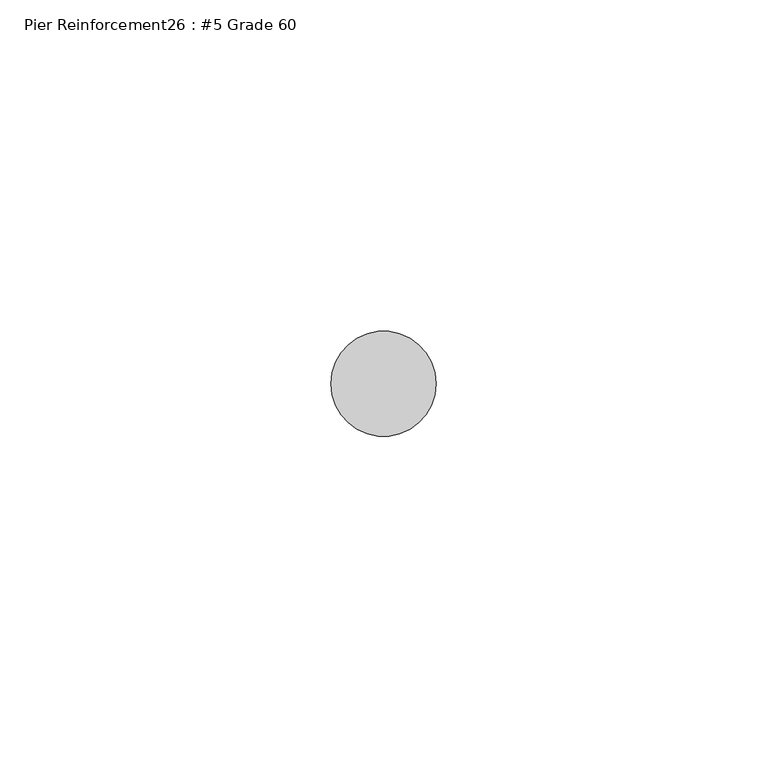
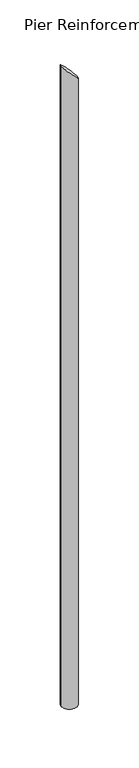
"""IFC4 building model written with IfcOpenShell, lengths in millimetres: proxy geometry, Pier Reinforcement26 : #5 Grade 60."""

import ifcopenshell
import ifcopenshell.guid

model = None  # the IFC model being written
_history = None  # IfcOwnerHistory: only IFC2X3 demands one
_inside = {}  # id of a spatial element -> (the spatial element, [elements in it])
_under = {}  # id of a project, library or spatial element -> (it, [spatial elements below it])
_declared = {}  # id of a project -> (the project, [libraries it declares])
_typed = {}  # id of a type object -> (the type object, [elements of that type])
_made_of = {}  # id of a material, layer set ... -> (it, [elements and type objects made of it])


def new_model(schema):
    """Start an empty IFC model of exactly this schema.

    Asked for "IFC4X3", IfcOpenShell would pick the latest addendum, in which some entities
    have other attributes; the version numbers below select the first issue.
    IFC2X3 requires an IfcOwnerHistory on every rooted entity: one is made here for all.
    """
    global model, _history
    if schema == "IFC4X3":
        model = ifcopenshell.file(schema_version=(4, 3, 0, 0))
    else:
        model = ifcopenshell.file(schema=schema)
    _inside.clear()
    _under.clear()
    _declared.clear()
    _typed.clear()
    _made_of.clear()
    _history = None
    if model.schema == "IFC2X3":
        org = make("IfcOrganization", Name="unknown")
        user = make(
            "IfcPersonAndOrganization",
            ThePerson=make("IfcPerson", FamilyName="unknown"),
            TheOrganization=org,
        )
        app = make(
            "IfcApplication",
            ApplicationDeveloper=org,
            Version="unknown",
            ApplicationFullName="unknown",
            ApplicationIdentifier="unknown",
        )
        _history = make(
            "IfcOwnerHistory",
            OwningUser=user,
            OwningApplication=app,
            ChangeAction="ADDED",
            CreationDate=0,
        )
    return model


def make(cls, **values):
    """One entity of the class cls with the attributes given. An attribute that is None is left unset."""
    return model.create_entity(
        cls, **{name: value for name, value in values.items() if value is not None}
    )


def rooted(cls, **values):
    """An entity with a GlobalId (a new one), such as an element, a storey or a relation."""
    return make(cls, GlobalId=ifcopenshell.guid.new(), OwnerHistory=_history, **values)


def si_unit(unit_type, name, prefix=None):
    """IfcSIUnit, for example si_unit("LENGTHUNIT", "METRE", prefix="MILLI")."""
    return make("IfcSIUnit", UnitType=unit_type, Prefix=prefix, Name=name)


def assignment(units):
    """IfcUnitAssignment: the units of a project."""
    return None if units is None else make("IfcUnitAssignment", Units=units)


def point(xyz):
    """IfcCartesianPoint."""
    return None if xyz is None else make("IfcCartesianPoint", Coordinates=xyz)


def direction(xyz):
    """IfcDirection."""
    return None if xyz is None else make("IfcDirection", DirectionRatios=xyz)


def frame(location, z_axis=None, x_axis=None):
    """IfcAxis2Placement3D, a coordinate frame: its origin and axes. An axis left out is left unset."""
    return make(
        "IfcAxis2Placement3D",
        Location=point(location),
        Axis=direction(z_axis),
        RefDirection=direction(x_axis),
    )


def origin():
    """The frame at (0, 0, 0) with its axes left unset."""
    return frame((0.0, 0.0, 0.0))


def place(relative_to, where):
    """IfcLocalPlacement: puts the frame where relative to a parent placement (None: the world)."""
    return make(
        "IfcLocalPlacement", PlacementRelTo=relative_to, RelativePlacement=where
    )


def context(
    kind, dimensions, precision=None, world=None, true_north=None, identifier=None
):
    """IfcGeometricRepresentationContext, for example the 3D "Model" context."""
    return make(
        "IfcGeometricRepresentationContext",
        ContextIdentifier=identifier,
        ContextType=kind,
        CoordinateSpaceDimension=dimensions,
        Precision=precision,
        WorldCoordinateSystem=world,
        TrueNorth=true_north,
    )


def project(units=None, contexts=None):
    """IfcProject with its units and contexts."""
    return rooted(
        "IfcProject",
        Name="project",
        RepresentationContexts=contexts,
        UnitsInContext=assignment(units),
    )


def spatial(cls, under=None, at=None, **own):
    """A site, building, storey or space (cls), placed at a placement, below another one or the project."""
    s = rooted(cls, ObjectPlacement=at, **own)
    if under is not None:
        _under.setdefault(under.id(), (under, []))[1].append(s)
    return s


def circle_curve(where, radius):
    """IfcCircle in the frame where."""
    return make("IfcCircle", Position=where, Radius=radius)


def ellipse_curve(where, semi_axis1, semi_axis2):
    """IfcEllipse in the frame where."""
    return make(
        "IfcEllipse", Position=where, SemiAxis1=semi_axis1, SemiAxis2=semi_axis2
    )


def shape(context_of_items, identifier, shape_type, items):
    """IfcShapeRepresentation: the items that make up one representation, for example the "Body"."""
    return make(
        "IfcShapeRepresentation",
        ContextOfItems=context_of_items,
        RepresentationIdentifier=identifier,
        RepresentationType=shape_type,
        Items=items,
    )


def source(mapping_origin, context_of_items, identifier, shape_type, items):
    """IfcRepresentationMap: a shape defined once, which mapped items show again and again."""
    return make(
        "IfcRepresentationMap",
        MappingOrigin=mapping_origin,
        MappedRepresentation=shape(context_of_items, identifier, shape_type, items),
    )


def transform(
    local_origin,
    x_axis=None,
    y_axis=None,
    z_axis=None,
    scale=None,
    scale2=None,
    scale3=None,
    uniform=True,
):
    """IfcCartesianTransformationOperator3D, or its non-uniform kind. x_axis, y_axis, z_axis: its Axis1, 2, 3."""
    if uniform:
        return make(
            "IfcCartesianTransformationOperator3D",
            Axis1=direction(x_axis),
            Axis2=direction(y_axis),
            LocalOrigin=point(local_origin),
            Scale=scale,
            Axis3=direction(z_axis),
        )
    return make(
        "IfcCartesianTransformationOperator3DnonUniform",
        Axis1=direction(x_axis),
        Axis2=direction(y_axis),
        LocalOrigin=point(local_origin),
        Scale=scale,
        Axis3=direction(z_axis),
        Scale2=scale2,
        Scale3=scale3,
    )


def mapped(mapping_source, mapping_target):
    """IfcMappedItem: shows the shape of a source again, moved by a transform."""
    return make(
        "IfcMappedItem", MappingSource=mapping_source, MappingTarget=mapping_target
    )


def made_of(thing, what):
    """Note that an element or type object is made of a material, layer set ...; save() writes the relation."""
    if what is not None:
        _made_of.setdefault(what.id(), (what, []))[1].append(thing)
    return thing


def element(
    cls,
    number,
    at=None,
    inside=None,
    cuts=None,
    type_object=None,
    material=None,
    context=None,
    identifier="Body",
    shape_type=None,
    held_by="IfcProductDefinitionShape",
    body=None,
    shapes=None,
    **own,
):
    """One element of the class cls, such as IfcWall. Its Tag is "e" and its number.

    at: its placement. inside: the storey or other place that contains it. cuts: it is an
    opening in that element (IfcRelVoidsElement). A single representation is given by context,
    identifier, shape_type and body (its items); several are given by shapes. held_by: the class
    of the entity that holds the representations. save() writes the other relations.
    """
    e = rooted(cls, Tag="e%d" % number, ObjectPlacement=at, **own)
    if body is not None:
        shapes = [shape(context, identifier, shape_type, body)]
    if shapes is not None:
        e.Representation = make(held_by, Representations=shapes)
    if inside is not None:
        _inside.setdefault(inside.id(), (inside, []))[1].append(e)
    if cuts is not None:
        rooted(
            "IfcRelVoidsElement", RelatingBuildingElement=cuts, RelatedOpeningElement=e
        )
    if type_object is not None:
        _typed.setdefault(type_object.id(), (type_object, []))[1].append(e)
    return made_of(e, material)


def aggregate(whole, parts):
    """IfcRelAggregates: a whole, such as a stair, and the parts it consists of."""
    return rooted("IfcRelAggregates", RelatingObject=whole, RelatedObjects=parts)


def save(model, path):
    """Write the relations noted so far, then the file.

    IfcRelAggregates (storeys below a building ...), IfcRelContainedInSpatialStructure (elements
    in a storey), IfcRelDefinesByType, IfcRelAssociatesMaterial and IfcRelDeclares: one each for
    every whole, place, type object, material and project.
    """
    for whole, parts in _under.values():
        aggregate(whole, parts)
    for where, things in _inside.values():
        rooted(
            "IfcRelContainedInSpatialStructure",
            RelatedElements=things,
            RelatingStructure=where,
        )
    for kind, things in _typed.values():
        rooted("IfcRelDefinesByType", RelatedObjects=things, RelatingType=kind)
    for what, things in _made_of.values():
        rooted("IfcRelAssociatesMaterial", RelatedObjects=things, RelatingMaterial=what)
    for by, libraries in _declared.values():
        rooted("IfcRelDeclares", RelatingContext=by, RelatedDefinitions=libraries)
    model.write(path)


def plane_surface(at):
    """IfcPlane: the flat surface through the origin of the frame at, square to its z axis."""
    return make("IfcPlane", Position=at)


def cylinder_surface(at, radius):
    """IfcCylindricalSurface: all points at the distance radius from the z axis of the frame at."""
    return make("IfcCylindricalSurface", Position=at, Radius=radius)


def advanced_brep(points, edges, surfaces, faces):
    """IfcAdvancedBrep: a solid bounded by faces that lie on surfaces and meet in shared edges.

    An edge is (start, end): straight between two places in points (the first is 0);
    or (start, end, curve); or (start, end, curve, False) where it runs against its curve.
    A face is (place in surfaces, loops), or (place, loops, False) where it looks against
    its surface's normal. A loop lists edges by number (the first is 1), with a minus sign
    where the edge is run from its end to its start. The first loop is the outer one.
    """
    corners = [point(p) for p in points]
    vertices = [make("IfcVertexPoint", VertexGeometry=c) for c in corners]
    made = []
    for start, end, *more in edges:
        made.append(
            make(
                "IfcEdgeCurve",
                EdgeStart=vertices[start],
                EdgeEnd=vertices[end],
                EdgeGeometry=more[0] if more else make("IfcPolyline", Points=[corners[start], corners[end]]),
                SameSense=more[1] if len(more) > 1 else True,
            )
        )
    hull = []
    for where, loops, *sense in faces:
        bounds = []
        for j, loop in enumerate(loops):
            ring = [make("IfcOrientedEdge", EdgeElement=made[abs(k) - 1], Orientation=k > 0) for k in loop]
            bounds.append(
                make(
                    "IfcFaceOuterBound" if j == 0 else "IfcFaceBound",
                    Bound=make("IfcEdgeLoop", EdgeList=ring),
                    Orientation=True,
                )
            )
        hull.append(make("IfcAdvancedFace", Bounds=bounds, FaceSurface=surfaces[where], SameSense=sense[0] if sense else True))
    return make("IfcAdvancedBrep", Outer=make("IfcClosedShell", CfsFaces=hull))


def pier_reinforcement26_5_grade_60_ff8834b7(model_context):
    return source(origin(), model_context, "Body", "AdvancedBrep", [
        advanced_brep(
        [(587484.5778122, -534096.6663841, -733.425), (587500.4528122, -534096.6663841, -733.425), (587500.4528122, -534096.6663841, -63.5), (587484.5778122, -534096.6663841, -47.625)],
        [
            (0, 1, circle_curve(frame((587492.5153122, -534096.6663841, -733.425), z_axis=(0.0, 0.0, -1.0), x_axis=(-1.0, 0.0, 0.0)), 7.9375)),
            (1, 0, circle_curve(frame((587492.5153122, -534096.6663841, -733.425), z_axis=(0.0, 0.0, -1.0), x_axis=(-1.0, 0.0, 0.0)), 7.9375)),
            (1, 2),
            (2, 3, ellipse_curve(frame((587492.5153122, -534096.6663841, -55.5625), z_axis=(-0.7071067811865458, 0.0, -0.7071067811865493), x_axis=(-0.7071067811865493, 0.0, 0.7071067811865456)), 11.2253202, 7.9375)),
            (3, 0),
            (3, 2, ellipse_curve(frame((587492.5153122, -534096.6663841, -55.5625), z_axis=(-0.7071067811865458, 0.0, -0.7071067811865493), x_axis=(-0.7071067811865493, 0.0, 0.7071067811865456)), 11.2253202, 7.9375)),
        ],
        [
            plane_surface(frame((587484.5778122, -534096.6663841, -733.425), z_axis=(0.0, 0.0, -1.0), x_axis=(0.0, 1.0, 0.0))),
            cylinder_surface(frame((587492.5153122, -534096.6663841, -733.425), z_axis=(0.0, 0.0, 1.0), x_axis=(-1.0, 0.0, 0.0)), 7.9375),
            plane_surface(frame((587484.5778122, -534071.2663841, -47.625), z_axis=(0.7071067811865458, 0.0, 0.7071067811865493), x_axis=(0.0, -1.0, 0.0))),
        ],
        [
            (0, [[1, 2]]),
            (1, [[-2, 3, 4, 5]]),
            (1, [[-1, -5, 6, -3]]),
            (2, [[-4, -6]]),
        ],
    ),
    ])


if __name__ == "__main__":
    model = new_model("IFC4")
    model_context = context("Model", 3, world=origin())
    ifc_project = project(units=[si_unit("LENGTHUNIT", "METRE", prefix="MILLI")], contexts=[model_context])
    site = spatial("IfcSite", under=ifc_project)
    building = spatial("IfcBuilding", under=site)
    placement = place(None, origin())
    pier_reinforcement26_5_grade_60_shape = pier_reinforcement26_5_grade_60_ff8834b7(model_context)
    element("IfcBuildingElementProxy", 1, Name="Pier Reinforcement26 : #5 Grade 60", ObjectType="Pier Reinforcement26 : #5 Grade 60", at=placement, inside=building, context=model_context, shape_type="MappedRepresentation", body=[
        mapped(pier_reinforcement26_5_grade_60_shape, transform((0.0, 0.0, 0.0), x_axis=(1.0, 0.0, 0.0), y_axis=(0.0, 1.0, 0.0), z_axis=(0.0, 0.0, 1.0))),
    ])
    save(model, "model.ifc")

# Revit data of these elements
# Element 1 (IfcBuildingElementProxy, "Pier Reinforcement26 : #5 Grade 60")
#   Materials on its faces: "#4 GR. 60 REINF. @ 16\" O.C. EW."
# Materials
#   "#4 GR. 60 REINF. @ 16\" O.C. EW.": class "Generic", colour RGB 84 83 81, transparency 0, Cost = 0
